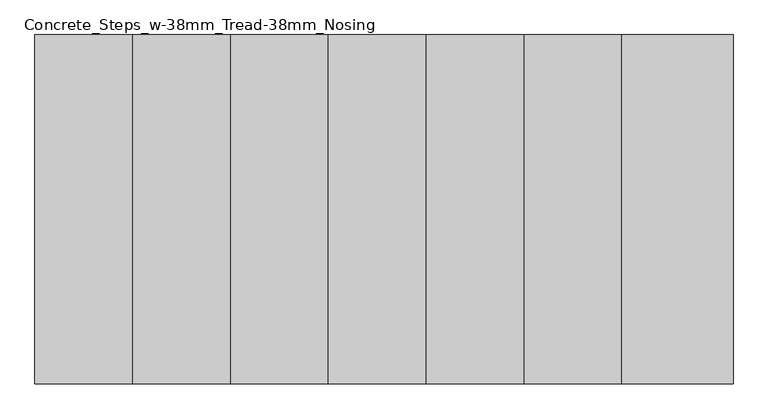
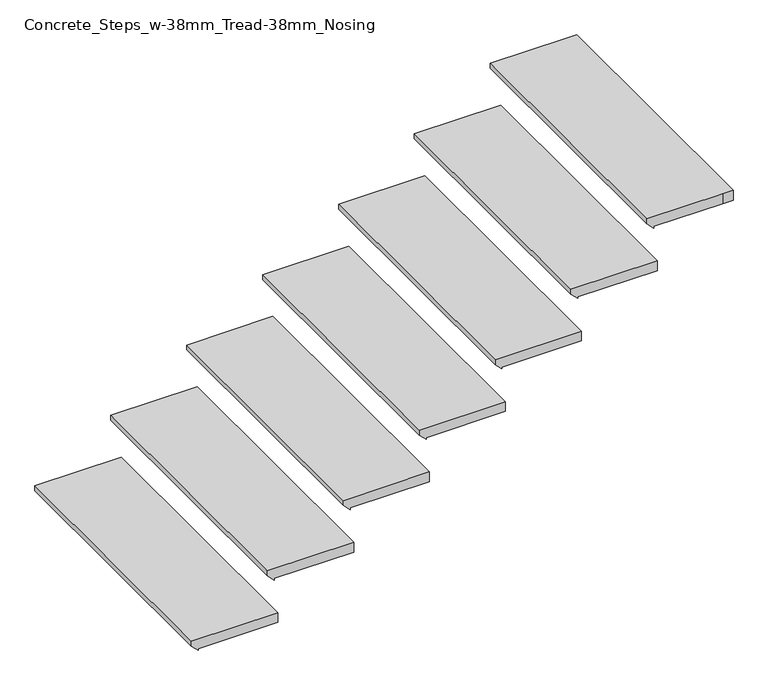
"""IFC4 building model written with IfcOpenShell, lengths in millimetres: stair flight geometry, Concrete_Steps_w-38mm_Tread-38mm_Nosing."""

from ifc_helpers import new_model, si_unit, origin, place, context, project, spatial, faceted_brep, source, transform, mapped, element, save


def concrete_steps_w_38mm_tread_38mm_nosing_129f34e4(model_context):
    return source(origin(), model_context, "Body", "Brep", [
        faceted_brep([(-5863.6361778, 8211.7063821, 157.4205882), (-5863.6361778, 8211.7063821, 176.4705882), (-5863.6361778, 9211.7063821, 176.4705882), (-5863.6361778, 9211.7063821, 157.4205882), (-5838.2361778, 8211.7063821, 132.0205882), (-5838.2361778, 9211.7063821, 132.0205882), (-5838.2361778, 9211.7063821, 138.4705882), (-5838.2361778, 8211.7063821, 138.4705882), (-5545.6361778, 8211.7063821, 176.4705882), (-5545.6361778, 9211.7063821, 176.4705882), (-5545.6361778, 9211.7063821, 138.4705882), (-5545.6361778, 8211.7063821, 138.4705882)], [[[0, 1, 2, 3]], [[4, 0, 3, 5]], [[4, 5, 6, 7]], [[2, 1, 8, 9]], [[6, 10, 11, 7]], [[2, 9, 10, 6, 5, 3]], [[8, 1, 0, 4, 7, 11]], [[9, 8, 11, 10]]]),
        faceted_brep([(-5583.6361778, 9211.7063821, 352.9411765), (-5583.6361778, 8211.7063821, 352.9411765), (-5265.6361778, 8211.7063821, 352.9411765), (-5265.6361778, 9211.7063821, 352.9411765), (-5558.2361778, 9211.7063821, 314.9411765), (-5265.6361778, 9211.7063821, 314.9411765), (-5265.6361778, 8211.7063821, 314.9411765), (-5558.2361778, 8211.7063821, 314.9411765), (-5558.2361778, 9211.7063821, 308.4911765), (-5583.6361778, 9211.7063821, 333.8911765), (-5583.6361778, 8211.7063821, 333.8911765), (-5558.2361778, 8211.7063821, 308.4911765)], [[[0, 1, 2, 3]], [[4, 5, 6, 7]], [[0, 3, 5, 4, 8, 9]], [[2, 1, 10, 11, 7, 6]], [[3, 2, 6, 5]], [[10, 1, 0, 9]], [[11, 10, 9, 8]], [[11, 8, 4, 7]]]),
        faceted_brep([(-5303.6361778, 9211.7063821, 529.4117647), (-5303.6361778, 8211.7063821, 529.4117647), (-4985.6361778, 8211.7063821, 529.4117647), (-4985.6361778, 9211.7063821, 529.4117647), (-5278.2361778, 9211.7063821, 491.4117647), (-4985.6361778, 9211.7063821, 491.4117647), (-4985.6361778, 8211.7063821, 491.4117647), (-5278.2361778, 8211.7063821, 491.4117647), (-5278.2361778, 9211.7063821, 484.9617647), (-5303.6361778, 9211.7063821, 510.3617647), (-5303.6361778, 8211.7063821, 510.3617647), (-5278.2361778, 8211.7063821, 484.9617647)], [[[0, 1, 2, 3]], [[4, 5, 6, 7]], [[0, 3, 5, 4, 8, 9]], [[2, 1, 10, 11, 7, 6]], [[3, 2, 6, 5]], [[10, 1, 0, 9]], [[11, 10, 9, 8]], [[11, 8, 4, 7]]]),
        faceted_brep([(-5023.6361778, 9211.7063821, 705.8823529), (-5023.6361778, 8211.7063821, 705.8823529), (-4705.6361778, 8211.7063821, 705.8823529), (-4705.6361778, 9211.7063821, 705.8823529), (-4998.2361778, 9211.7063821, 667.8823529), (-4705.6361778, 9211.7063821, 667.8823529), (-4705.6361778, 8211.7063821, 667.8823529), (-4998.2361778, 8211.7063821, 667.8823529), (-4998.2361778, 9211.7063821, 661.4323529), (-5023.6361778, 9211.7063821, 686.8323529), (-5023.6361778, 8211.7063821, 686.8323529), (-4998.2361778, 8211.7063821, 661.4323529)], [[[0, 1, 2, 3]], [[4, 5, 6, 7]], [[0, 3, 5, 4, 8, 9]], [[2, 1, 10, 11, 7, 6]], [[3, 2, 6, 5]], [[10, 1, 0, 9]], [[11, 10, 9, 8]], [[11, 8, 4, 7]]]),
        faceted_brep([(-4743.6361778, 9211.7063821, 882.3529412), (-4743.6361778, 8211.7063821, 882.3529412), (-4425.6361778, 8211.7063821, 882.3529412), (-4425.6361778, 9211.7063821, 882.3529412), (-4718.2361778, 9211.7063821, 844.3529412), (-4425.6361778, 9211.7063821, 844.3529412), (-4425.6361778, 8211.7063821, 844.3529412), (-4718.2361778, 8211.7063821, 844.3529412), (-4718.2361778, 9211.7063821, 837.9029412), (-4743.6361778, 9211.7063821, 863.3029412), (-4743.6361778, 8211.7063821, 863.3029412), (-4718.2361778, 8211.7063821, 837.9029412)], [[[0, 1, 2, 3]], [[4, 5, 6, 7]], [[0, 3, 5, 4, 8, 9]], [[2, 1, 10, 11, 7, 6]], [[3, 2, 6, 5]], [[10, 1, 0, 9]], [[11, 10, 9, 8]], [[11, 8, 4, 7]]]),
        faceted_brep([(-4463.6361778, 9211.7063821, 1058.8235294), (-4463.6361778, 8211.7063821, 1058.8235294), (-4145.6361778, 8211.7063821, 1058.8235294), (-4145.6361778, 9211.7063821, 1058.8235294), (-4438.2361778, 9211.7063821, 1020.8235294), (-4145.6361778, 9211.7063821, 1020.8235294), (-4145.6361778, 8211.7063821, 1020.8235294), (-4438.2361778, 8211.7063821, 1020.8235294), (-4438.2361778, 9211.7063821, 1014.3735294), (-4463.6361778, 9211.7063821, 1039.7735294), (-4463.6361778, 8211.7063821, 1039.7735294), (-4438.2361778, 8211.7063821, 1014.3735294)], [[[0, 1, 2, 3]], [[4, 5, 6, 7]], [[0, 3, 5, 4, 8, 9]], [[2, 1, 10, 11, 7, 6]], [[3, 2, 6, 5]], [[10, 1, 0, 9]], [[11, 10, 9, 8]], [[11, 8, 4, 7]]]),
        faceted_brep([(-3865.6361778, 9211.7063821, 1235.2941176), (-3903.6361778, 9211.7063821, 1235.2941176), (-4183.6361778, 9211.7063821, 1235.2941176), (-4183.6361778, 8211.7063821, 1235.2941176), (-3903.6361778, 8211.7063821, 1235.2941176), (-3865.6361778, 8211.7063821, 1235.2941176), (-3903.6361778, 9211.7063821, 1197.2941176), (-3865.6361778, 9211.7063821, 1197.2941176), (-3865.6361778, 8211.7063821, 1197.2941176), (-3903.6361778, 8211.7063821, 1197.2941176), (-4158.2361778, 8211.7063821, 1197.2941176), (-4158.2361778, 9211.7063821, 1197.2941176), (-4158.2361778, 9211.7063821, 1190.8441176), (-4183.6361778, 9211.7063821, 1216.2441176), (-4183.6361778, 8211.7063821, 1216.2441176), (-4158.2361778, 8211.7063821, 1190.8441176)], [[[0, 1, 2, 3, 4, 5]], [[6, 7, 8, 9, 10, 11]], [[1, 0, 7, 6]], [[2, 1, 6, 11, 12, 13]], [[4, 3, 14, 15, 10, 9]], [[5, 4, 9, 8]], [[0, 5, 8, 7]], [[14, 3, 2, 13]], [[15, 14, 13, 12]], [[15, 12, 11, 10]]]),
    ])


if __name__ == "__main__":
    model = new_model("IFC4")
    model_context = context("Model", 3, world=origin())
    ifc_project = project(units=[si_unit("LENGTHUNIT", "METRE", prefix="MILLI")], contexts=[model_context])
    site = spatial("IfcSite", under=ifc_project)
    building = spatial("IfcBuilding", under=site)
    placement = place(None, origin())
    concrete_steps_w_38mm_tread_38mm_nosing_shape = concrete_steps_w_38mm_tread_38mm_nosing_129f34e4(model_context)
    element("IfcStairFlight", 1, ObjectType="Concrete_Steps_w-38mm_Tread-38mm_Nosing", at=placement, inside=building, context=model_context, shape_type="MappedRepresentation", body=[
        mapped(concrete_steps_w_38mm_tread_38mm_nosing_shape, transform((0.0, 0.0, 0.0), x_axis=(1.0, 0.0, 0.0), y_axis=(0.0, 1.0, 0.0), z_axis=(0.0, 0.0, 1.0))),
    ])
    save(model, "model.ifc")

# Revit data of these elements
# Element 1 (IfcStairFlight, "Concrete_Steps_w-38mm_Tread-38mm_Nosing")
#   Materials on its faces: "Concrete, Cast-in-Place gray"
# Materials
#   "Concrete, Cast-in-Place gray": class "Concrete", colour RGB 192 192 192, transparency 0, Description = "Cast-in-place concrete", Cost = 0
